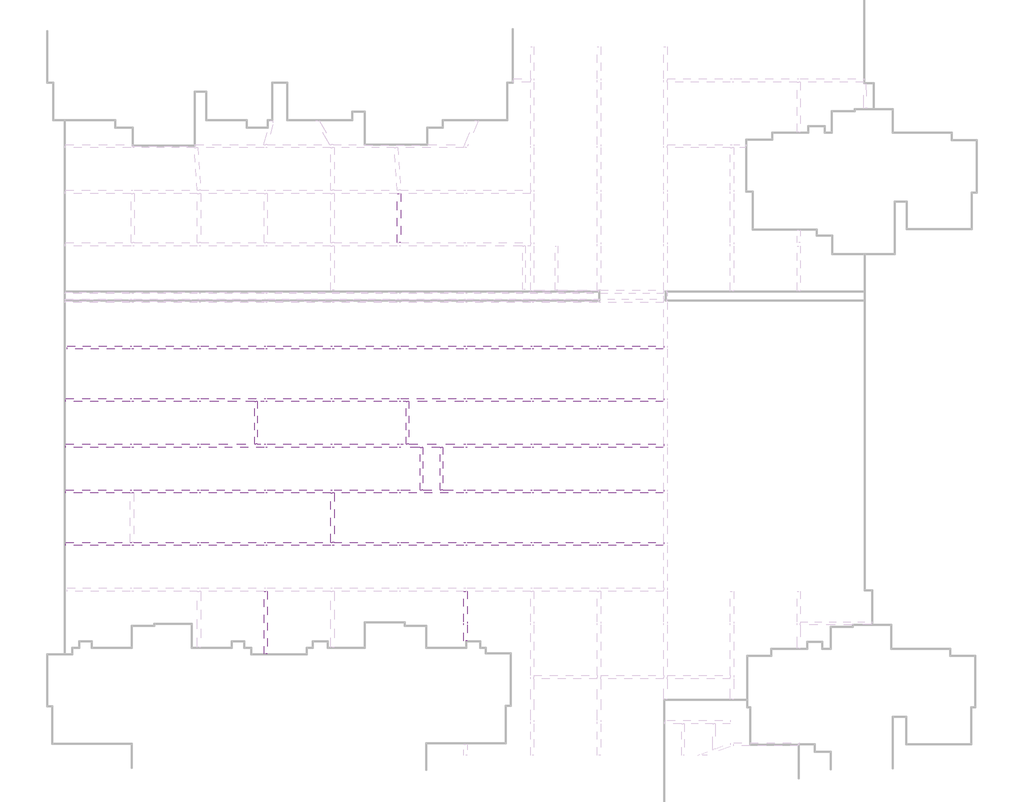
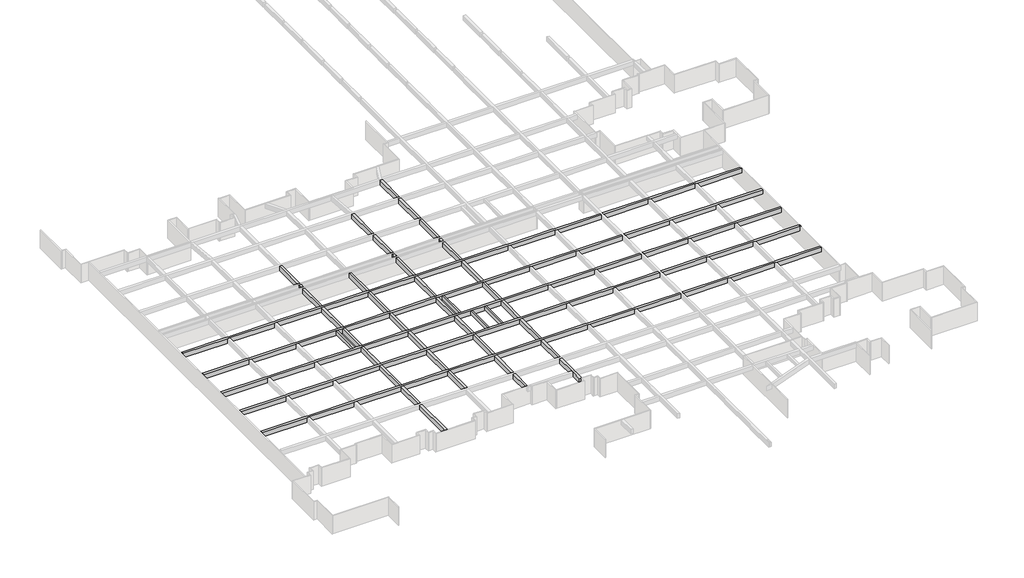
# One storey, part 9 of 14: 13 beams.
"""IFC4 building model written with IfcOpenShell, lengths in millimetres."""

from ifc_helpers import new_model, si_unit, frame, origin, place, context, project, spatial, polyline, outline, extrude, faceted_brep, element, save

model = new_model("IFC4")

# Units and contexts
model_context = context("Model", 3, world=origin())
ifc_project = project(units=[si_unit("LENGTHUNIT", "METRE", prefix="MILLI")], contexts=[model_context])

# Site, building, storey
site = spatial("IfcSite", under=ifc_project)
building = spatial("IfcBuilding", under=site)
storey = spatial("IfcBuildingStorey", under=building, Name="户型图", Elevation=0.0)

# Beams
placement = place(None, origin())
element("IfcBeam", 1, ObjectType="混凝土 - 矩形梁 : KL_beam", at=placement, inside=storey, context=model_context, shape_type="Brep", body=[
    faceted_brep([(-593917.6529954, -134659.4327531, 3300.0), (-593917.6529954, -134659.4327531, 2500.0), (-593917.6529954, -135059.4327531, 2500.0), (-593917.6529954, -135059.4327531, 3300.0), (-522267.6529954, -134659.4327531, 3300.0), (-522267.6529954, -135059.4327531, 3300.0), (-522267.6529954, -135059.4327531, 2500.0), (-522267.6529954, -134659.4327531, 2500.0), (-586331.2602569, -135059.4327531, 3300.0), (-585931.2602569, -135059.4327531, 3300.0), (-578267.6529954, -135059.4327531, 3300.0), (-577867.6529954, -135059.4327531, 3300.0), (-570267.6529954, -135059.4327531, 3300.0), (-569867.6529954, -135059.4327531, 3300.0), (-562267.6529954, -135059.4327531, 3300.0), (-561867.6529954, -135059.4327531, 3300.0), (-554267.6529954, -135059.4327531, 3300.0), (-553867.6529954, -135059.4327531, 3300.0), (-546267.6529954, -135059.4327531, 3300.0), (-545867.6529954, -135059.4327531, 3300.0), (-538267.6529954, -135059.4327531, 3300.0), (-537867.6529954, -135059.4327531, 3300.0), (-530267.6529954, -135059.4327531, 3300.0), (-529867.6529954, -135059.4327531, 3300.0), (-529867.6529954, -134659.4327531, 3300.0), (-530267.6529954, -134659.4327531, 3300.0), (-537867.6529954, -134659.4327531, 3300.0), (-538267.6529954, -134659.4327531, 3300.0), (-545867.6529954, -134659.4327531, 3300.0), (-546267.6529954, -134659.4327531, 3300.0), (-553867.6529954, -134659.4327531, 3300.0), (-554267.6529954, -134659.4327531, 3300.0), (-561867.6529954, -134659.4327531, 3300.0), (-562267.6529954, -134659.4327531, 3300.0), (-569867.6529954, -134659.4327531, 3300.0), (-570267.6529954, -134659.4327531, 3300.0), (-577867.6529954, -134659.4327531, 3300.0), (-578267.6529954, -134659.4327531, 3300.0), (-585931.2602569, -134659.4327531, 3300.0), (-586331.2602569, -134659.4327531, 3300.0), (-586331.2602569, -135059.4327531, 2500.0), (-585931.2602569, -135059.4327531, 2500.0), (-578267.6529954, -135059.4327531, 2500.0), (-577867.6529954, -135059.4327531, 2500.0), (-570267.6529954, -135059.4327531, 2500.0), (-569867.6529954, -135059.4327531, 2500.0), (-562267.6529954, -135059.4327531, 2500.0), (-561867.6529954, -135059.4327531, 2500.0), (-554267.6529954, -135059.4327531, 2500.0), (-553867.6529954, -135059.4327531, 2500.0), (-546267.6529954, -135059.4327531, 2500.0), (-545867.6529954, -135059.4327531, 2500.0), (-538267.6529954, -135059.4327531, 2500.0), (-537867.6529954, -135059.4327531, 2500.0), (-530267.6529954, -135059.4327531, 2500.0), (-529867.6529954, -135059.4327531, 2500.0), (-586331.2602569, -134659.4327531, 2500.0), (-585931.2602569, -134659.4327531, 2500.0), (-578267.6529954, -134659.4327531, 2500.0), (-577867.6529954, -134659.4327531, 2500.0), (-570267.6529954, -134659.4327531, 2500.0), (-569867.6529954, -134659.4327531, 2500.0), (-562267.6529954, -134659.4327531, 2500.0), (-561867.6529954, -134659.4327531, 2500.0), (-554267.6529954, -134659.4327531, 2500.0), (-553867.6529954, -134659.4327531, 2500.0), (-546267.6529954, -134659.4327531, 2500.0), (-545867.6529954, -134659.4327531, 2500.0), (-538267.6529954, -134659.4327531, 2500.0), (-537867.6529954, -134659.4327531, 2500.0), (-530267.6529954, -134659.4327531, 2500.0), (-529867.6529954, -134659.4327531, 2500.0)], [[[0, 1, 2, 3]], [[4, 5, 6, 7]], [[0, 3, 8, 9, 10, 11, 12, 13, 14, 15, 16, 17, 18, 19, 20, 21, 22, 23, 5, 4, 24, 25, 26, 27, 28, 29, 30, 31, 32, 33, 34, 35, 36, 37, 38, 39]], [[3, 2, 40, 41, 42, 43, 44, 45, 46, 47, 48, 49, 50, 51, 52, 53, 54, 55, 6, 5, 23, 22, 21, 20, 19, 18, 17, 16, 15, 14, 13, 12, 11, 10, 9, 8]], [[2, 1, 56, 57, 58, 59, 60, 61, 62, 63, 64, 65, 66, 67, 68, 69, 70, 71, 7, 6, 55, 54, 53, 52, 51, 50, 49, 48, 47, 46, 45, 44, 43, 42, 41, 40]], [[1, 0, 39, 38, 37, 36, 35, 34, 33, 32, 31, 30, 29, 28, 27, 26, 25, 24, 4, 7, 71, 70, 69, 68, 67, 66, 65, 64, 63, 62, 61, 60, 59, 58, 57, 56]]]),
    faceted_brep([(-498227.6529954, -135059.4327531, 3300.0), (-498227.6529954, -134659.4327531, 3300.0), (-505867.6529954, -134659.4327531, 3300.0), (-506267.6529954, -134659.4327531, 3300.0), (-513867.6529954, -134659.4327531, 3300.0), (-514267.6529954, -134659.4327531, 3300.0), (-521867.6529954, -134659.4327531, 3300.0), (-521867.6529954, -135059.4327531, 3300.0), (-514267.6529954, -135059.4327531, 3300.0), (-513867.6529954, -135059.4327531, 3300.0), (-506267.6529954, -135059.4327531, 3300.0), (-505867.6529954, -135059.4327531, 3300.0), (-498227.6529954, -135059.4327531, 2500.0), (-521867.6529954, -135059.4327531, 2500.0), (-514267.6529954, -135059.4327531, 2500.0), (-513867.6529954, -135059.4327531, 2500.0), (-506267.6529954, -135059.4327531, 2500.0), (-505867.6529954, -135059.4327531, 2500.0), (-498227.6529954, -134659.4327531, 2500.0), (-521867.6529954, -134659.4327531, 2500.0), (-514267.6529954, -134659.4327531, 2500.0), (-513867.6529954, -134659.4327531, 2500.0), (-506267.6529954, -134659.4327531, 2500.0), (-505867.6529954, -134659.4327531, 2500.0)], [[[0, 1, 2, 3, 4, 5, 6, 7, 8, 9, 10, 11]], [[12, 0, 11, 10, 9, 8, 7, 13, 14, 15, 16, 17]], [[18, 12, 17, 16, 15, 14, 13, 19, 20, 21, 22, 23]], [[1, 18, 23, 22, 21, 20, 19, 6, 5, 4, 3, 2]], [[1, 0, 12, 18]], [[7, 6, 19, 13]]]),
])
element("IfcBeam", 2, ObjectType="混凝土 - 矩形梁 : KL_beam", at=placement, inside=storey, context=model_context, shape_type="Brep", body=[
    faceted_brep([(-594067.6529954, -141359.4327531, 3300.0), (-594067.6529954, -140959.4327531, 3300.0), (-594067.6529954, -140959.4327531, 2500.0), (-594067.6529954, -141359.4327531, 2500.0), (-586331.2602569, -141359.4327531, 3300.0), (-585931.2602569, -141359.4327531, 3300.0), (-578267.6529954, -141359.4327531, 3300.0), (-577867.6529954, -141359.4327531, 3300.0), (-571417.6529954, -141359.4327531, 3300.0), (-571117.6529954, -141359.4327531, 3300.0), (-570267.6529954, -141359.4327531, 3300.0), (-569867.6529954, -141359.4327531, 3300.0), (-562267.6529954, -141359.4327531, 3300.0), (-561867.6529954, -141359.4327531, 3300.0), (-554267.6529954, -141359.4327531, 3300.0), (-553867.6529954, -141359.4327531, 3300.0), (-553217.6529954, -141359.4327531, 3300.0), (-552917.6529954, -141359.4327531, 3300.0), (-546267.6529954, -141359.4327531, 3300.0), (-545867.6529954, -141359.4327531, 3300.0), (-538267.6529954, -141359.4327531, 3300.0), (-537867.6529954, -141359.4327531, 3300.0), (-530267.6529954, -141359.4327531, 3300.0), (-529867.6529954, -141359.4327531, 3300.0), (-522267.6529954, -141359.4327531, 3300.0), (-522267.6529954, -140959.4327531, 3300.0), (-529867.6529954, -140959.4327531, 3300.0), (-530267.6529954, -140959.4327531, 3300.0), (-537867.6529954, -140959.4327531, 3300.0), (-538267.6529954, -140959.4327531, 3300.0), (-545867.6529954, -140959.4327531, 3300.0), (-546267.6529954, -140959.4327531, 3300.0), (-553867.6529954, -140959.4327531, 3300.0), (-554267.6529954, -140959.4327531, 3300.0), (-561867.6529954, -140959.4327531, 3300.0), (-562267.6529954, -140959.4327531, 3300.0), (-569867.6529954, -140959.4327531, 3300.0), (-570267.6529954, -140959.4327531, 3300.0), (-577867.6529954, -140959.4327531, 3300.0), (-578267.6529954, -140959.4327531, 3300.0), (-585931.2602569, -140959.4327531, 3300.0), (-586331.2602569, -140959.4327531, 3300.0), (-522267.6529954, -140959.4327531, 2500.0), (-529867.6529954, -140959.4327531, 2500.0), (-530267.6529954, -140959.4327531, 2500.0), (-537867.6529954, -140959.4327531, 2500.0), (-538267.6529954, -140959.4327531, 2500.0), (-545867.6529954, -140959.4327531, 2500.0), (-546267.6529954, -140959.4327531, 2500.0), (-553867.6529954, -140959.4327531, 2500.0), (-554267.6529954, -140959.4327531, 2500.0), (-561867.6529954, -140959.4327531, 2500.0), (-562267.6529954, -140959.4327531, 2500.0), (-569867.6529954, -140959.4327531, 2500.0), (-570267.6529954, -140959.4327531, 2500.0), (-577867.6529954, -140959.4327531, 2500.0), (-578267.6529954, -140959.4327531, 2500.0), (-585931.2602569, -140959.4327531, 2500.0), (-586331.2602569, -140959.4327531, 2500.0), (-522267.6529954, -141359.4327531, 2500.0), (-529867.6529954, -141359.4327531, 2500.0), (-530267.6529954, -141359.4327531, 2500.0), (-537867.6529954, -141359.4327531, 2500.0), (-538267.6529954, -141359.4327531, 2500.0), (-545867.6529954, -141359.4327531, 2500.0), (-546267.6529954, -141359.4327531, 2500.0), (-553867.6529954, -141359.4327531, 2500.0), (-554267.6529954, -141359.4327531, 2500.0), (-561867.6529954, -141359.4327531, 2500.0), (-562267.6529954, -141359.4327531, 2500.0), (-569867.6529954, -141359.4327531, 2500.0), (-570267.6529954, -141359.4327531, 2500.0), (-577867.6529954, -141359.4327531, 2500.0), (-578267.6529954, -141359.4327531, 2500.0), (-585931.2602569, -141359.4327531, 2500.0), (-586331.2602569, -141359.4327531, 2500.0)], [[[0, 1, 2, 3]], [[1, 0, 4, 5, 6, 7, 8, 9, 10, 11, 12, 13, 14, 15, 16, 17, 18, 19, 20, 21, 22, 23, 24, 25, 26, 27, 28, 29, 30, 31, 32, 33, 34, 35, 36, 37, 38, 39, 40, 41]], [[2, 1, 41, 40, 39, 38, 37, 36, 35, 34, 33, 32, 31, 30, 29, 28, 27, 26, 25, 42, 43, 44, 45, 46, 47, 48, 49, 50, 51, 52, 53, 54, 55, 56, 57, 58]], [[3, 2, 58, 57, 56, 55, 54, 53, 52, 51, 50, 49, 48, 47, 46, 45, 44, 43, 42, 59, 60, 61, 62, 63, 64, 65, 66, 67, 68, 69, 70, 71, 72, 73, 74, 75]], [[0, 3, 75, 74, 73, 72, 71, 70, 69, 68, 67, 66, 65, 64, 63, 62, 61, 60, 59, 24, 23, 22, 21, 20, 19, 18, 17, 16, 15, 14, 13, 12, 11, 10, 9, 8, 7, 6, 5, 4]], [[25, 24, 59, 42]]]),
    faceted_brep([(-498227.6529954, -140959.4327531, 3300.0), (-498227.6529954, -141359.4327531, 3300.0), (-498227.6529954, -141359.4327531, 2500.0), (-498227.6529954, -140959.4327531, 2500.0), (-521867.6529954, -141359.4327531, 3300.0), (-521867.6529954, -140959.4327531, 3300.0), (-521867.6529954, -140959.4327531, 2500.0), (-521867.6529954, -141359.4327531, 2500.0), (-505867.6529954, -140959.4327531, 3300.0), (-506267.6529954, -140959.4327531, 3300.0), (-513867.6529954, -140959.4327531, 3300.0), (-514267.6529954, -140959.4327531, 3300.0), (-514267.6529954, -141359.4327531, 3300.0), (-513867.6529954, -141359.4327531, 3300.0), (-506267.6529954, -141359.4327531, 3300.0), (-505867.6529954, -141359.4327531, 3300.0), (-505867.6529954, -140959.4327531, 2500.0), (-506267.6529954, -140959.4327531, 2500.0), (-513867.6529954, -140959.4327531, 2500.0), (-514267.6529954, -140959.4327531, 2500.0), (-505867.6529954, -141359.4327531, 2500.0), (-506267.6529954, -141359.4327531, 2500.0), (-513867.6529954, -141359.4327531, 2500.0), (-514267.6529954, -141359.4327531, 2500.0)], [[[0, 1, 2, 3]], [[4, 5, 6, 7]], [[1, 0, 8, 9, 10, 11, 5, 4, 12, 13, 14, 15]], [[0, 3, 16, 17, 18, 19, 6, 5, 11, 10, 9, 8]], [[3, 2, 20, 21, 22, 23, 7, 6, 19, 18, 17, 16]], [[2, 1, 15, 14, 13, 12, 4, 7, 23, 22, 21, 20]]]),
])
element("IfcBeam", 3, ObjectType="混凝土 - 矩形梁 : KL_beam", at=placement, inside=storey, context=model_context, shape_type="Brep", body=[
    faceted_brep([(-594067.6529954, -146459.4327531, 3300.0), (-594067.6529954, -146459.4327531, 2500.0), (-594067.6529954, -146859.4327531, 2500.0), (-594067.6529954, -146859.4327531, 3300.0), (-522267.6529954, -146459.4327531, 3300.0), (-522267.6529954, -146859.4327531, 3300.0), (-522267.6529954, -146859.4327531, 2500.0), (-522267.6529954, -146459.4327531, 2500.0), (-586331.2602569, -146859.4327531, 3300.0), (-585931.2602569, -146859.4327531, 3300.0), (-578267.6529954, -146859.4327531, 3300.0), (-577867.6529954, -146859.4327531, 3300.0), (-570267.6529954, -146859.4327531, 3300.0), (-569867.6529954, -146859.4327531, 3300.0), (-562267.6529954, -146859.4327531, 3300.0), (-561867.6529954, -146859.4327531, 3300.0), (-554267.6529954, -146859.4327531, 3300.0), (-553867.6529954, -146859.4327531, 3300.0), (-551517.6529954, -146859.4327531, 3300.0), (-551217.6529954, -146859.4327531, 3300.0), (-549117.6529954, -146859.4327531, 3300.0), (-548817.6529954, -146859.4327531, 3300.0), (-546267.6529954, -146859.4327531, 3300.0), (-545867.6529954, -146859.4327531, 3300.0), (-538267.6529954, -146859.4327531, 3300.0), (-537867.6529954, -146859.4327531, 3300.0), (-530267.6529954, -146859.4327531, 3300.0), (-529867.6529954, -146859.4327531, 3300.0), (-529867.6529954, -146459.4327531, 3300.0), (-530267.6529954, -146459.4327531, 3300.0), (-537867.6529954, -146459.4327531, 3300.0), (-538267.6529954, -146459.4327531, 3300.0), (-545867.6529954, -146459.4327531, 3300.0), (-546267.6529954, -146459.4327531, 3300.0), (-552917.6529954, -146459.4327531, 3300.0), (-553217.6529954, -146459.4327531, 3300.0), (-553867.6529954, -146459.4327531, 3300.0), (-554267.6529954, -146459.4327531, 3300.0), (-561867.6529954, -146459.4327531, 3300.0), (-562267.6529954, -146459.4327531, 3300.0), (-569867.6529954, -146459.4327531, 3300.0), (-570267.6529954, -146459.4327531, 3300.0), (-571117.6529954, -146459.4327531, 3300.0), (-571417.6529954, -146459.4327531, 3300.0), (-577867.6529954, -146459.4327531, 3300.0), (-578267.6529954, -146459.4327531, 3300.0), (-585931.2602569, -146459.4327531, 3300.0), (-586331.2602569, -146459.4327531, 3300.0), (-586331.2602569, -146859.4327531, 2500.0), (-585931.2602569, -146859.4327531, 2500.0), (-578267.6529954, -146859.4327531, 2500.0), (-577867.6529954, -146859.4327531, 2500.0), (-570267.6529954, -146859.4327531, 2500.0), (-569867.6529954, -146859.4327531, 2500.0), (-562267.6529954, -146859.4327531, 2500.0), (-561867.6529954, -146859.4327531, 2500.0), (-554267.6529954, -146859.4327531, 2500.0), (-553867.6529954, -146859.4327531, 2500.0), (-546267.6529954, -146859.4327531, 2500.0), (-545867.6529954, -146859.4327531, 2500.0), (-538267.6529954, -146859.4327531, 2500.0), (-537867.6529954, -146859.4327531, 2500.0), (-530267.6529954, -146859.4327531, 2500.0), (-529867.6529954, -146859.4327531, 2500.0), (-586331.2602569, -146459.4327531, 2500.0), (-585931.2602569, -146459.4327531, 2500.0), (-578267.6529954, -146459.4327531, 2500.0), (-577867.6529954, -146459.4327531, 2500.0), (-570267.6529954, -146459.4327531, 2500.0), (-569867.6529954, -146459.4327531, 2500.0), (-562267.6529954, -146459.4327531, 2500.0), (-561867.6529954, -146459.4327531, 2500.0), (-554267.6529954, -146459.4327531, 2500.0), (-553867.6529954, -146459.4327531, 2500.0), (-546267.6529954, -146459.4327531, 2500.0), (-545867.6529954, -146459.4327531, 2500.0), (-538267.6529954, -146459.4327531, 2500.0), (-537867.6529954, -146459.4327531, 2500.0), (-530267.6529954, -146459.4327531, 2500.0), (-529867.6529954, -146459.4327531, 2500.0)], [[[0, 1, 2, 3]], [[4, 5, 6, 7]], [[0, 3, 8, 9, 10, 11, 12, 13, 14, 15, 16, 17, 18, 19, 20, 21, 22, 23, 24, 25, 26, 27, 5, 4, 28, 29, 30, 31, 32, 33, 34, 35, 36, 37, 38, 39, 40, 41, 42, 43, 44, 45, 46, 47]], [[3, 2, 48, 49, 50, 51, 52, 53, 54, 55, 56, 57, 58, 59, 60, 61, 62, 63, 6, 5, 27, 26, 25, 24, 23, 22, 21, 20, 19, 18, 17, 16, 15, 14, 13, 12, 11, 10, 9, 8]], [[2, 1, 64, 65, 66, 67, 68, 69, 70, 71, 72, 73, 74, 75, 76, 77, 78, 79, 7, 6, 63, 62, 61, 60, 59, 58, 57, 56, 55, 54, 53, 52, 51, 50, 49, 48]], [[1, 0, 47, 46, 45, 44, 43, 42, 41, 40, 39, 38, 37, 36, 35, 34, 33, 32, 31, 30, 29, 28, 4, 7, 79, 78, 77, 76, 75, 74, 73, 72, 71, 70, 69, 68, 67, 66, 65, 64]]]),
    faceted_brep([(-498227.6529954, -146859.4327531, 3300.0), (-498227.6529954, -146459.4327531, 3300.0), (-505867.6529954, -146459.4327531, 3300.0), (-506267.6529954, -146459.4327531, 3300.0), (-513867.6529954, -146459.4327531, 3300.0), (-514267.6529954, -146459.4327531, 3300.0), (-521867.6529954, -146459.4327531, 3300.0), (-521867.6529954, -146859.4327531, 3300.0), (-514267.6529954, -146859.4327531, 3300.0), (-513867.6529954, -146859.4327531, 3300.0), (-506267.6529954, -146859.4327531, 3300.0), (-505867.6529954, -146859.4327531, 3300.0), (-498227.6529954, -146859.4327531, 2500.0), (-521867.6529954, -146859.4327531, 2500.0), (-514267.6529954, -146859.4327531, 2500.0), (-513867.6529954, -146859.4327531, 2500.0), (-506267.6529954, -146859.4327531, 2500.0), (-505867.6529954, -146859.4327531, 2500.0), (-498227.6529954, -146459.4327531, 2500.0), (-521867.6529954, -146459.4327531, 2500.0), (-514267.6529954, -146459.4327531, 2500.0), (-513867.6529954, -146459.4327531, 2500.0), (-506267.6529954, -146459.4327531, 2500.0), (-505867.6529954, -146459.4327531, 2500.0)], [[[0, 1, 2, 3, 4, 5, 6, 7, 8, 9, 10, 11]], [[12, 0, 11, 10, 9, 8, 7, 13, 14, 15, 16, 17]], [[18, 12, 17, 16, 15, 14, 13, 19, 20, 21, 22, 23]], [[1, 18, 23, 22, 21, 20, 19, 6, 5, 4, 3, 2]], [[1, 0, 12, 18]], [[7, 6, 19, 13]]]),
])
element("IfcBeam", 4, ObjectType="混凝土 - 矩形梁 : KL_beam", at=placement, inside=storey, context=model_context, shape_type="Brep", body=[
    faceted_brep([(-498067.6529954, -151959.4327531, 3300.0), (-498067.6529954, -152359.4327531, 3300.0), (-498067.6529954, -152359.4327531, 2500.0), (-498067.6529954, -151959.4327531, 2500.0), (-498107.6529954, -151959.4327531, 3300.0), (-498107.6529954, -152359.4327531, 3300.0), (-498107.6529954, -152359.4327531, 2500.0), (-498107.6529954, -151959.4327531, 2500.0)], [[[0, 1, 2, 3]], [[1, 0, 4, 5]], [[2, 1, 5, 6]], [[3, 2, 6, 7]], [[0, 3, 7, 4]], [[5, 4, 7, 6]]]),
    faceted_brep([(-594067.6529954, -151959.4327531, 3300.0), (-594067.6529954, -151959.4327531, 2500.0), (-594067.6529954, -152359.4327531, 2500.0), (-594067.6529954, -152359.4327531, 3300.0), (-522267.6529954, -151959.4327531, 3300.0), (-522267.6529954, -152359.4327531, 3300.0), (-522267.6529954, -152359.4327531, 2500.0), (-522267.6529954, -151959.4327531, 2500.0), (-586331.2602569, -152359.4327531, 3300.0), (-585931.2602569, -152359.4327531, 3300.0), (-578267.6529954, -152359.4327531, 3300.0), (-577867.6529954, -152359.4327531, 3300.0), (-570267.6529954, -152359.4327531, 3300.0), (-569867.6529954, -152359.4327531, 3300.0), (-562267.6529954, -152359.4327531, 3300.0), (-561867.6529954, -152359.4327531, 3300.0), (-554267.6529954, -152359.4327531, 3300.0), (-553867.6529954, -152359.4327531, 3300.0), (-546267.6529954, -152359.4327531, 3300.0), (-545867.6529954, -152359.4327531, 3300.0), (-538267.6529954, -152359.4327531, 3300.0), (-537867.6529954, -152359.4327531, 3300.0), (-530267.6529954, -152359.4327531, 3300.0), (-529867.6529954, -152359.4327531, 3300.0), (-529867.6529954, -151959.4327531, 3300.0), (-530267.6529954, -151959.4327531, 3300.0), (-537867.6529954, -151959.4327531, 3300.0), (-538267.6529954, -151959.4327531, 3300.0), (-545867.6529954, -151959.4327531, 3300.0), (-546267.6529954, -151959.4327531, 3300.0), (-548817.6529954, -151959.4327531, 3300.0), (-549117.6529954, -151959.4327531, 3300.0), (-551217.6529954, -151959.4327531, 3300.0), (-551517.6529954, -151959.4327531, 3300.0), (-553867.6529954, -151959.4327531, 3300.0), (-554267.6529954, -151959.4327531, 3300.0), (-561867.6529954, -151959.4327531, 3300.0), (-562267.6529954, -151959.4327531, 3300.0), (-569867.6529954, -151959.4327531, 3300.0), (-570267.6529954, -151959.4327531, 3300.0), (-577867.6529954, -151959.4327531, 3300.0), (-578267.6529954, -151959.4327531, 3300.0), (-585931.2602569, -151959.4327531, 3300.0), (-586331.2602569, -151959.4327531, 3300.0), (-586331.2602569, -152359.4327531, 2500.0), (-585931.2602569, -152359.4327531, 2500.0), (-578267.6529954, -152359.4327531, 2500.0), (-577867.6529954, -152359.4327531, 2500.0), (-570267.6529954, -152359.4327531, 2500.0), (-569867.6529954, -152359.4327531, 2500.0), (-562267.6529954, -152359.4327531, 2500.0), (-561867.6529954, -152359.4327531, 2500.0), (-554267.6529954, -152359.4327531, 2500.0), (-553867.6529954, -152359.4327531, 2500.0), (-546267.6529954, -152359.4327531, 2500.0), (-545867.6529954, -152359.4327531, 2500.0), (-538267.6529954, -152359.4327531, 2500.0), (-537867.6529954, -152359.4327531, 2500.0), (-530267.6529954, -152359.4327531, 2500.0), (-529867.6529954, -152359.4327531, 2500.0), (-586331.2602569, -151959.4327531, 2500.0), (-585931.2602569, -151959.4327531, 2500.0), (-578267.6529954, -151959.4327531, 2500.0), (-577867.6529954, -151959.4327531, 2500.0), (-570267.6529954, -151959.4327531, 2500.0), (-569867.6529954, -151959.4327531, 2500.0), (-562267.6529954, -151959.4327531, 2500.0), (-561867.6529954, -151959.4327531, 2500.0), (-554267.6529954, -151959.4327531, 2500.0), (-553867.6529954, -151959.4327531, 2500.0), (-546267.6529954, -151959.4327531, 2500.0), (-545867.6529954, -151959.4327531, 2500.0), (-538267.6529954, -151959.4327531, 2500.0), (-537867.6529954, -151959.4327531, 2500.0), (-530267.6529954, -151959.4327531, 2500.0), (-529867.6529954, -151959.4327531, 2500.0)], [[[0, 1, 2, 3]], [[4, 5, 6, 7]], [[0, 3, 8, 9, 10, 11, 12, 13, 14, 15, 16, 17, 18, 19, 20, 21, 22, 23, 5, 4, 24, 25, 26, 27, 28, 29, 30, 31, 32, 33, 34, 35, 36, 37, 38, 39, 40, 41, 42, 43]], [[3, 2, 44, 45, 46, 47, 48, 49, 50, 51, 52, 53, 54, 55, 56, 57, 58, 59, 6, 5, 23, 22, 21, 20, 19, 18, 17, 16, 15, 14, 13, 12, 11, 10, 9, 8]], [[2, 1, 60, 61, 62, 63, 64, 65, 66, 67, 68, 69, 70, 71, 72, 73, 74, 75, 7, 6, 59, 58, 57, 56, 55, 54, 53, 52, 51, 50, 49, 48, 47, 46, 45, 44]], [[1, 0, 43, 42, 41, 40, 39, 38, 37, 36, 35, 34, 33, 32, 31, 30, 29, 28, 27, 26, 25, 24, 4, 7, 75, 74, 73, 72, 71, 70, 69, 68, 67, 66, 65, 64, 63, 62, 61, 60]]]),
    faceted_brep([(-521867.6529954, -152359.4327531, 3300.0), (-521867.6529954, -151959.4327531, 3300.0), (-521867.6529954, -151959.4327531, 2500.0), (-521867.6529954, -152359.4327531, 2500.0), (-498227.6529954, -151959.4327531, 3300.0), (-498227.6529954, -152359.4327531, 3300.0), (-498227.6529954, -152359.4327531, 2500.0), (-498227.6529954, -151959.4327531, 2500.0), (-514267.6529954, -152359.4327531, 3300.0), (-513867.6529954, -152359.4327531, 3300.0), (-506267.6529954, -152359.4327531, 3300.0), (-505867.6529954, -152359.4327531, 3300.0), (-505867.6529954, -151959.4327531, 3300.0), (-506267.6529954, -151959.4327531, 3300.0), (-513867.6529954, -151959.4327531, 3300.0), (-514267.6529954, -151959.4327531, 3300.0), (-514267.6529954, -152359.4327531, 2500.0), (-513867.6529954, -152359.4327531, 2500.0), (-506267.6529954, -152359.4327531, 2500.0), (-505867.6529954, -152359.4327531, 2500.0), (-514267.6529954, -151959.4327531, 2500.0), (-513867.6529954, -151959.4327531, 2500.0), (-506267.6529954, -151959.4327531, 2500.0), (-505867.6529954, -151959.4327531, 2500.0)], [[[0, 1, 2, 3]], [[4, 5, 6, 7]], [[1, 0, 8, 9, 10, 11, 5, 4, 12, 13, 14, 15]], [[0, 3, 16, 17, 18, 19, 6, 5, 11, 10, 9, 8]], [[3, 2, 20, 21, 22, 23, 7, 6, 19, 18, 17, 16]], [[2, 1, 15, 14, 13, 12, 4, 7, 23, 22, 21, 20]]]),
])
element("IfcBeam", 5, ObjectType="混凝土 - 矩形梁 : KL_beam", at=placement, inside=storey, context=model_context, shape_type="Brep", body=[
    faceted_brep([(-594067.6529954, -158659.4327531, 3300.0), (-594067.6529954, -158259.4327531, 3300.0), (-594067.6529954, -158259.4327531, 2500.0), (-594067.6529954, -158659.4327531, 2500.0), (-586331.2602569, -158659.4327531, 3300.0), (-585931.2602569, -158659.4327531, 3300.0), (-578267.6529954, -158659.4327531, 3300.0), (-577867.6529954, -158659.4327531, 3300.0), (-570267.6529954, -158659.4327531, 3300.0), (-569867.6529954, -158659.4327531, 3300.0), (-562267.6529954, -158659.4327531, 3300.0), (-561867.6529954, -158659.4327531, 3300.0), (-554267.6529954, -158659.4327531, 3300.0), (-553867.6529954, -158659.4327531, 3300.0), (-546267.6529954, -158659.4327531, 3300.0), (-545867.6529954, -158659.4327531, 3300.0), (-538267.6529954, -158659.4327531, 3300.0), (-537867.6529954, -158659.4327531, 3300.0), (-530267.6529954, -158659.4327531, 3300.0), (-529867.6529954, -158659.4327531, 3300.0), (-522267.6529954, -158659.4327531, 3300.0), (-522267.6529954, -158259.4327531, 3300.0), (-529867.6529954, -158259.4327531, 3300.0), (-530267.6529954, -158259.4327531, 3300.0), (-537867.6529954, -158259.4327531, 3300.0), (-538267.6529954, -158259.4327531, 3300.0), (-545867.6529954, -158259.4327531, 3300.0), (-546267.6529954, -158259.4327531, 3300.0), (-553867.6529954, -158259.4327531, 3300.0), (-554267.6529954, -158259.4327531, 3300.0), (-561867.6529954, -158259.4327531, 3300.0), (-562267.6529954, -158259.4327531, 3300.0), (-569867.6529954, -158259.4327531, 3300.0), (-570267.6529954, -158259.4327531, 3300.0), (-577867.6529954, -158259.4327531, 3300.0), (-578267.6529954, -158259.4327531, 3300.0), (-585931.2602569, -158259.4327531, 3300.0), (-586331.2602569, -158259.4327531, 3300.0), (-522267.6529954, -158259.4327531, 2500.0), (-529867.6529954, -158259.4327531, 2500.0), (-530267.6529954, -158259.4327531, 2500.0), (-537867.6529954, -158259.4327531, 2500.0), (-538267.6529954, -158259.4327531, 2500.0), (-545867.6529954, -158259.4327531, 2500.0), (-546267.6529954, -158259.4327531, 2500.0), (-553867.6529954, -158259.4327531, 2500.0), (-554267.6529954, -158259.4327531, 2500.0), (-561867.6529954, -158259.4327531, 2500.0), (-562267.6529954, -158259.4327531, 2500.0), (-569867.6529954, -158259.4327531, 2500.0), (-570267.6529954, -158259.4327531, 2500.0), (-577867.6529954, -158259.4327531, 2500.0), (-578267.6529954, -158259.4327531, 2500.0), (-585931.2602569, -158259.4327531, 2500.0), (-586331.2602569, -158259.4327531, 2500.0), (-522267.6529954, -158659.4327531, 2500.0), (-529867.6529954, -158659.4327531, 2500.0), (-530267.6529954, -158659.4327531, 2500.0), (-537867.6529954, -158659.4327531, 2500.0), (-538267.6529954, -158659.4327531, 2500.0), (-545867.6529954, -158659.4327531, 2500.0), (-546267.6529954, -158659.4327531, 2500.0), (-553867.6529954, -158659.4327531, 2500.0), (-554267.6529954, -158659.4327531, 2500.0), (-561867.6529954, -158659.4327531, 2500.0), (-562267.6529954, -158659.4327531, 2500.0), (-569867.6529954, -158659.4327531, 2500.0), (-570267.6529954, -158659.4327531, 2500.0), (-577867.6529954, -158659.4327531, 2500.0), (-578267.6529954, -158659.4327531, 2500.0), (-585931.2602569, -158659.4327531, 2500.0), (-586331.2602569, -158659.4327531, 2500.0)], [[[0, 1, 2, 3]], [[1, 0, 4, 5, 6, 7, 8, 9, 10, 11, 12, 13, 14, 15, 16, 17, 18, 19, 20, 21, 22, 23, 24, 25, 26, 27, 28, 29, 30, 31, 32, 33, 34, 35, 36, 37]], [[2, 1, 37, 36, 35, 34, 33, 32, 31, 30, 29, 28, 27, 26, 25, 24, 23, 22, 21, 38, 39, 40, 41, 42, 43, 44, 45, 46, 47, 48, 49, 50, 51, 52, 53, 54]], [[3, 2, 54, 53, 52, 51, 50, 49, 48, 47, 46, 45, 44, 43, 42, 41, 40, 39, 38, 55, 56, 57, 58, 59, 60, 61, 62, 63, 64, 65, 66, 67, 68, 69, 70, 71]], [[0, 3, 71, 70, 69, 68, 67, 66, 65, 64, 63, 62, 61, 60, 59, 58, 57, 56, 55, 20, 19, 18, 17, 16, 15, 14, 13, 12, 11, 10, 9, 8, 7, 6, 5, 4]], [[21, 20, 55, 38]]]),
    faceted_brep([(-498227.6529954, -158259.4327531, 3300.0), (-498227.6529954, -158659.4327531, 3300.0), (-498227.6529954, -158659.4327531, 2500.0), (-498227.6529954, -158259.4327531, 2500.0), (-521867.6529954, -158659.4327531, 3300.0), (-521867.6529954, -158259.4327531, 3300.0), (-521867.6529954, -158259.4327531, 2500.0), (-521867.6529954, -158659.4327531, 2500.0), (-505867.6529954, -158259.4327531, 3300.0), (-506267.6529954, -158259.4327531, 3300.0), (-513867.6529954, -158259.4327531, 3300.0), (-514267.6529954, -158259.4327531, 3300.0), (-514267.6529954, -158659.4327531, 3300.0), (-513867.6529954, -158659.4327531, 3300.0), (-506267.6529954, -158659.4327531, 3300.0), (-505867.6529954, -158659.4327531, 3300.0), (-505867.6529954, -158259.4327531, 2500.0), (-506267.6529954, -158259.4327531, 2500.0), (-513867.6529954, -158259.4327531, 2500.0), (-514267.6529954, -158259.4327531, 2500.0), (-505867.6529954, -158659.4327531, 2500.0), (-506267.6529954, -158659.4327531, 2500.0), (-513867.6529954, -158659.4327531, 2500.0), (-514267.6529954, -158659.4327531, 2500.0)], [[[0, 1, 2, 3]], [[4, 5, 6, 7]], [[1, 0, 8, 9, 10, 11, 5, 4, 12, 13, 14, 15]], [[0, 3, 16, 17, 18, 19, 6, 5, 11, 10, 9, 8]], [[3, 2, 20, 21, 22, 23, 7, 6, 19, 18, 17, 16]], [[2, 1, 15, 14, 13, 12, 4, 7, 23, 22, 21, 20]]]),
])
element("IfcBeam", 6, ObjectType="混凝土 - 矩形梁 : KL_beam", at=placement, inside=storey, context=model_context, shape_type="SweptSolid", body=[
    extrude(outline(polyline([(-569867.6529954, -171682.856538), (-570267.6529954, -171682.856538), (-570267.6529954, -164159.4327531), (-569867.6529954, -164159.4327531), (-569867.6529954, -171682.856538)])), frame((0.0, 0.0, 2500.0), z_axis=(0.0, 0.0, 1.0), x_axis=(1.0, 0.0, 0.0)), (0.0, 0.0, 1.0), 800.0),
    extrude(outline(polyline([(-570267.6529954, -122659.4327531), (-569867.6529954, -122659.4327531), (-569867.6529954, -127959.4327532), (-570267.6529954, -127959.4327532), (-570267.6529954, -122659.4327531)])), frame((0.0, 0.0, 2500.0), z_axis=(0.0, 0.0, 1.0), x_axis=(1.0, 0.0, 0.0)), (0.0, 0.0, 1.0), 800.0),
    extrude(outline(polyline([(-570267.6529954, -128359.4327532), (-569867.6529954, -128359.4327532), (-569867.6529954, -129034.4327531), (-570267.6529954, -129034.4327531), (-570267.6529954, -128359.4327532)])), frame((0.0, 0.0, 2500.0), z_axis=(0.0, 0.0, 1.0), x_axis=(1.0, 0.0, 0.0)), (0.0, 0.0, 1.0), 800.0),
    extrude(outline(polyline([(-570267.6529954, -129434.4327531), (-569867.6529954, -129434.4327531), (-569867.6529954, -134659.4327531), (-570267.6529954, -134659.4327531), (-570267.6529954, -129434.4327531)])), frame((0.0, 0.0, 2500.0), z_axis=(0.0, 0.0, 1.0), x_axis=(1.0, 0.0, 0.0)), (0.0, 0.0, 1.0), 800.0),
    extrude(outline(polyline([(-570267.6529954, -135059.4327531), (-569867.6529954, -135059.4327531), (-569867.6529954, -140959.4327531), (-570267.6529954, -140959.4327531), (-570267.6529954, -135059.4327531)])), frame((0.0, 0.0, 2500.0), z_axis=(0.0, 0.0, 1.0), x_axis=(1.0, 0.0, 0.0)), (0.0, 0.0, 1.0), 800.0),
    extrude(outline(polyline([(-570267.6529954, -141359.4327531), (-569867.6529954, -141359.4327531), (-569867.6529954, -146459.4327531), (-570267.6529954, -146459.4327531), (-570267.6529954, -141359.4327531)])), frame((0.0, 0.0, 2500.0), z_axis=(0.0, 0.0, 1.0), x_axis=(1.0, 0.0, 0.0)), (0.0, 0.0, 1.0), 800.0),
    extrude(outline(polyline([(-570267.6529954, -146859.4327531), (-569867.6529954, -146859.4327531), (-569867.6529954, -151959.4327531), (-570267.6529954, -151959.4327531), (-570267.6529954, -146859.4327531)])), frame((0.0, 0.0, 2500.0), z_axis=(0.0, 0.0, 1.0), x_axis=(1.0, 0.0, 0.0)), (0.0, 0.0, 1.0), 800.0),
    extrude(outline(polyline([(-570267.6529954, -152359.4327531), (-569867.6529954, -152359.4327531), (-569867.6529954, -158259.4327531), (-570267.6529954, -158259.4327531), (-570267.6529954, -152359.4327531)])), frame((0.0, 0.0, 2500.0), z_axis=(0.0, 0.0, 1.0), x_axis=(1.0, 0.0, 0.0)), (0.0, 0.0, 1.0), 800.0),
    extrude(outline(polyline([(-570267.6529954, -158659.4327531), (-569867.6529954, -158659.4327531), (-569867.6529954, -163759.4327531), (-570267.6529954, -163759.4327531), (-570267.6529954, -158659.4327531)])), frame((0.0, 0.0, 2500.0), z_axis=(0.0, 0.0, 1.0), x_axis=(1.0, 0.0, 0.0)), (0.0, 0.0, 1.0), 800.0),
])
element("IfcBeam", 7, ObjectType="混凝土 - 矩形梁 : KL_beam", at=placement, inside=storey, context=model_context, shape_type="Brep", body=[
    faceted_brep([(-553867.6529954, -116357.5126628, 3300.0), (-554267.6529954, -116357.5126628, 3300.0), (-554267.6529954, -122259.4327531, 3300.0), (-553867.6529954, -122259.4327531, 3300.0), (-554267.6529954, -116357.5126628, 2500.0), (-554267.6529954, -122259.4327531, 2500.0), (-553867.6529954, -116357.5126628, 2500.0), (-553867.6529954, -122259.4327531, 2500.0)], [[[0, 1, 2, 3]], [[1, 4, 5, 2]], [[4, 6, 7, 5]], [[6, 0, 3, 7]], [[1, 0, 6, 4]], [[3, 2, 5, 7]]]),
    faceted_brep([(-553867.6529954, -167832.8565288, 3300.0), (-554267.6529954, -167832.8565288, 3300.0), (-554267.6529954, -167832.8565288, 2500.0), (-553867.6529954, -167832.8565288, 2500.0), (-554267.6529954, -164159.4327531, 3300.0), (-553867.6529954, -164159.4327531, 3300.0), (-553867.6529954, -164159.4327531, 2500.0), (-554267.6529954, -164159.4327531, 2500.0), (-553867.6529954, -167800.507479, 3300.0), (-553867.6529954, -167800.507479, 2500.0)], [[[0, 1, 2, 3]], [[4, 5, 6, 7]], [[1, 0, 8, 5, 4]], [[2, 1, 4, 7]], [[3, 2, 7, 6, 9]], [[0, 3, 9, 6, 5, 8]]]),
    faceted_brep([(-554267.6529954, -122659.4327531, 3300.0), (-553867.6529954, -122659.4327531, 3300.0), (-553867.6529954, -122659.4327531, 2500.0), (-554267.6529954, -122659.4327531, 2500.0), (-553867.6529954, -127959.4327532, 3300.0), (-554267.6529954, -127959.4327532, 3300.0), (-554267.6529954, -127959.4327532, 2500.0), (-553867.6529954, -127959.4327532, 2500.0)], [[[0, 1, 2, 3]], [[4, 5, 6, 7]], [[1, 0, 5, 4]], [[0, 3, 6, 5]], [[3, 2, 7, 6]], [[2, 1, 4, 7]]]),
    faceted_brep([(-553867.6529954, -128359.4327532, 3300.0), (-554267.6529954, -128359.4327532, 3300.0), (-554267.6529954, -129034.4327531, 3300.0), (-553867.6529954, -129034.4327531, 3300.0), (-554267.6529954, -128359.4327532, 2500.0), (-554267.6529954, -129034.4327531, 2500.0), (-553867.6529954, -128359.4327532, 2500.0), (-553867.6529954, -129034.4327531, 2500.0)], [[[0, 1, 2, 3]], [[1, 4, 5, 2]], [[4, 6, 7, 5]], [[6, 0, 3, 7]], [[1, 0, 6, 4]], [[3, 2, 5, 7]]]),
    faceted_brep([(-554267.6529954, -129434.4327531, 3300.0), (-553867.6529954, -129434.4327531, 3300.0), (-553867.6529954, -129434.4327531, 2500.0), (-554267.6529954, -129434.4327531, 2500.0), (-553867.6529954, -134659.4327531, 3300.0), (-554267.6529954, -134659.4327531, 3300.0), (-554267.6529954, -134659.4327531, 2500.0), (-553867.6529954, -134659.4327531, 2500.0)], [[[0, 1, 2, 3]], [[4, 5, 6, 7]], [[1, 0, 5, 4]], [[0, 3, 6, 5]], [[3, 2, 7, 6]], [[2, 1, 4, 7]]]),
    faceted_brep([(-553867.6529954, -135059.4327531, 3300.0), (-554267.6529954, -135059.4327531, 3300.0), (-554267.6529954, -140959.4327531, 3300.0), (-553867.6529954, -140959.4327531, 3300.0), (-554267.6529954, -135059.4327531, 2500.0), (-554267.6529954, -140959.4327531, 2500.0), (-553867.6529954, -135059.4327531, 2500.0), (-553867.6529954, -140959.4327531, 2500.0)], [[[0, 1, 2, 3]], [[1, 4, 5, 2]], [[4, 6, 7, 5]], [[6, 0, 3, 7]], [[1, 0, 6, 4]], [[3, 2, 5, 7]]]),
    faceted_brep([(-554267.6529954, -141359.4327531, 3300.0), (-553867.6529954, -141359.4327531, 3300.0), (-553867.6529954, -141359.4327531, 2500.0), (-554267.6529954, -141359.4327531, 2500.0), (-553867.6529954, -146459.4327531, 3300.0), (-554267.6529954, -146459.4327531, 3300.0), (-554267.6529954, -146459.4327531, 2500.0), (-553867.6529954, -146459.4327531, 2500.0)], [[[0, 1, 2, 3]], [[4, 5, 6, 7]], [[1, 0, 5, 4]], [[0, 3, 6, 5]], [[3, 2, 7, 6]], [[2, 1, 4, 7]]]),
    faceted_brep([(-553867.6529954, -146859.4327531, 3300.0), (-554267.6529954, -146859.4327531, 3300.0), (-554267.6529954, -151959.4327531, 3300.0), (-553867.6529954, -151959.4327531, 3300.0), (-554267.6529954, -146859.4327531, 2500.0), (-554267.6529954, -151959.4327531, 2500.0), (-553867.6529954, -146859.4327531, 2500.0), (-553867.6529954, -151959.4327531, 2500.0)], [[[0, 1, 2, 3]], [[1, 4, 5, 2]], [[4, 6, 7, 5]], [[6, 0, 3, 7]], [[1, 0, 6, 4]], [[3, 2, 5, 7]]]),
    faceted_brep([(-554267.6529954, -152359.4327531, 3300.0), (-553867.6529954, -152359.4327531, 3300.0), (-553867.6529954, -152359.4327531, 2500.0), (-554267.6529954, -152359.4327531, 2500.0), (-553867.6529954, -158259.4327531, 3300.0), (-554267.6529954, -158259.4327531, 3300.0), (-554267.6529954, -158259.4327531, 2500.0), (-553867.6529954, -158259.4327531, 2500.0)], [[[0, 1, 2, 3]], [[4, 5, 6, 7]], [[1, 0, 5, 4]], [[0, 3, 6, 5]], [[3, 2, 7, 6]], [[2, 1, 4, 7]]]),
    faceted_brep([(-553867.6529954, -158659.4327531, 3300.0), (-554267.6529954, -158659.4327531, 3300.0), (-554267.6529954, -163759.4327531, 3300.0), (-553867.6529954, -163759.4327531, 3300.0), (-554267.6529954, -158659.4327531, 2500.0), (-554267.6529954, -163759.4327531, 2500.0), (-553867.6529954, -158659.4327531, 2500.0), (-553867.6529954, -163759.4327531, 2500.0)], [[[0, 1, 2, 3]], [[1, 4, 5, 2]], [[4, 6, 7, 5]], [[6, 0, 3, 7]], [[1, 0, 6, 4]], [[3, 2, 5, 7]]]),
])
element("IfcBeam", 8, ObjectType="混凝土 - 矩形梁 : KL_beam", at=placement, inside=storey, context=model_context, shape_type="Brep", body=[
    faceted_brep([(-546267.6529954, -170082.6446455, 3300.0), (-546267.6529954, -170082.6446455, 2500.0), (-545867.6529954, -170082.6446455, 2500.0), (-545867.6529954, -170082.6446455, 3300.0), (-545867.6529954, -164159.4327531, 3300.0), (-545867.6529954, -164159.4327531, 2500.0), (-546267.6529954, -164159.4327531, 2500.0), (-546267.6529954, -164159.4327531, 3300.0), (-545867.6529954, -168200.507479, 2500.0), (-545867.6529954, -167800.507479, 2500.0), (-545867.6529954, -167800.507479, 3300.0), (-545867.6529954, -168200.507479, 3300.0), (-546267.6529954, -167800.507479, 3300.0), (-546267.6529954, -168200.507479, 3300.0), (-546267.6529954, -168200.507479, 2500.0), (-546267.6529954, -167800.507479, 2500.0)], [[[0, 1, 2, 3]], [[4, 5, 6, 7]], [[3, 2, 8, 9, 5, 4, 10, 11]], [[0, 3, 11, 10, 4, 7, 12, 13]], [[2, 1, 14, 15, 6, 5, 9, 8]], [[1, 0, 13, 12, 7, 6, 15, 14]]]),
    faceted_brep([(-545867.6529954, -110859.4327531, 2500.0), (-545867.6529954, -110859.4327531, 3300.0), (-545867.6529954, -115957.5126628, 3300.0), (-545867.6529954, -115957.5126628, 2500.0), (-545935.2758832, -110859.4327531, 3300.0), (-546267.6529954, -110859.4327531, 3300.0), (-546267.6529954, -115957.5126628, 3300.0), (-546267.6529954, -110859.4327531, 2500.0), (-545935.2758832, -110859.4327531, 2500.0), (-546267.6529954, -115957.5126628, 2500.0)], [[[0, 1, 2, 3]], [[1, 4, 5, 6, 2]], [[7, 8, 0, 3, 9]], [[5, 7, 9, 6]], [[1, 0, 8, 7, 5, 4]], [[3, 2, 6, 9]]]),
    faceted_brep([(-545867.6529954, -116357.5126628, 3300.0), (-545867.6529954, -116357.5126628, 2500.0), (-546267.6529954, -116357.5126628, 2500.0), (-546267.6529954, -116357.5126628, 3300.0), (-545867.6529954, -122259.4327531, 3300.0), (-545867.6529954, -122259.4327531, 2500.0), (-546267.6529954, -122259.4327531, 3300.0), (-546267.6529954, -122259.4327531, 2500.0)], [[[0, 1, 2, 3]], [[1, 0, 4, 5]], [[0, 3, 6, 4]], [[2, 1, 5, 7]], [[3, 2, 7, 6]], [[5, 4, 6, 7]]]),
    faceted_brep([(-545867.6529954, -122659.4327531, 3300.0), (-545867.6529954, -122659.4327531, 2500.0), (-546267.6529954, -122659.4327531, 2500.0), (-546267.6529954, -122659.4327531, 3300.0), (-545867.6529954, -127959.4327532, 3300.0), (-545867.6529954, -127959.4327532, 2500.0), (-546267.6529954, -127959.4327532, 3300.0), (-546267.6529954, -127959.4327532, 2500.0)], [[[0, 1, 2, 3]], [[1, 0, 4, 5]], [[0, 3, 6, 4]], [[2, 1, 5, 7]], [[3, 2, 7, 6]], [[5, 4, 6, 7]]]),
    faceted_brep([(-545867.6529954, -128359.4327532, 3300.0), (-545867.6529954, -128359.4327532, 2500.0), (-546267.6529954, -128359.4327532, 2500.0), (-546267.6529954, -128359.4327532, 3300.0), (-545867.6529954, -129034.4327531, 3300.0), (-545867.6529954, -129034.4327531, 2500.0), (-546267.6529954, -129034.4327531, 3300.0), (-546267.6529954, -129034.4327531, 2500.0)], [[[0, 1, 2, 3]], [[1, 0, 4, 5]], [[0, 3, 6, 4]], [[2, 1, 5, 7]], [[3, 2, 7, 6]], [[5, 4, 6, 7]]]),
    faceted_brep([(-545867.6529954, -129434.4327531, 3300.0), (-545867.6529954, -129434.4327531, 2500.0), (-546267.6529954, -129434.4327531, 2500.0), (-546267.6529954, -129434.4327531, 3300.0), (-545867.6529954, -134659.4327531, 3300.0), (-545867.6529954, -134659.4327531, 2500.0), (-546267.6529954, -134659.4327531, 3300.0), (-546267.6529954, -134659.4327531, 2500.0)], [[[0, 1, 2, 3]], [[1, 0, 4, 5]], [[0, 3, 6, 4]], [[2, 1, 5, 7]], [[3, 2, 7, 6]], [[5, 4, 6, 7]]]),
    faceted_brep([(-545867.6529954, -135059.4327531, 3300.0), (-545867.6529954, -135059.4327531, 2500.0), (-546267.6529954, -135059.4327531, 2500.0), (-546267.6529954, -135059.4327531, 3300.0), (-545867.6529954, -140959.4327531, 3300.0), (-545867.6529954, -140959.4327531, 2500.0), (-546267.6529954, -140959.4327531, 3300.0), (-546267.6529954, -140959.4327531, 2500.0)], [[[0, 1, 2, 3]], [[1, 0, 4, 5]], [[0, 3, 6, 4]], [[2, 1, 5, 7]], [[3, 2, 7, 6]], [[5, 4, 6, 7]]]),
    faceted_brep([(-545867.6529954, -141359.4327531, 3300.0), (-545867.6529954, -141359.4327531, 2500.0), (-546267.6529954, -141359.4327531, 2500.0), (-546267.6529954, -141359.4327531, 3300.0), (-545867.6529954, -146459.4327531, 3300.0), (-545867.6529954, -146459.4327531, 2500.0), (-546267.6529954, -146459.4327531, 3300.0), (-546267.6529954, -146459.4327531, 2500.0)], [[[0, 1, 2, 3]], [[1, 0, 4, 5]], [[0, 3, 6, 4]], [[2, 1, 5, 7]], [[3, 2, 7, 6]], [[5, 4, 6, 7]]]),
    faceted_brep([(-545867.6529954, -146859.4327531, 3300.0), (-545867.6529954, -146859.4327531, 2500.0), (-546267.6529954, -146859.4327531, 2500.0), (-546267.6529954, -146859.4327531, 3300.0), (-545867.6529954, -151959.4327531, 3300.0), (-545867.6529954, -151959.4327531, 2500.0), (-546267.6529954, -151959.4327531, 3300.0), (-546267.6529954, -151959.4327531, 2500.0)], [[[0, 1, 2, 3]], [[1, 0, 4, 5]], [[0, 3, 6, 4]], [[2, 1, 5, 7]], [[3, 2, 7, 6]], [[5, 4, 6, 7]]]),
    faceted_brep([(-545867.6529954, -152359.4327531, 3300.0), (-545867.6529954, -152359.4327531, 2500.0), (-546267.6529954, -152359.4327531, 2500.0), (-546267.6529954, -152359.4327531, 3300.0), (-545867.6529954, -158259.4327531, 3300.0), (-545867.6529954, -158259.4327531, 2500.0), (-546267.6529954, -158259.4327531, 3300.0), (-546267.6529954, -158259.4327531, 2500.0)], [[[0, 1, 2, 3]], [[1, 0, 4, 5]], [[0, 3, 6, 4]], [[2, 1, 5, 7]], [[3, 2, 7, 6]], [[5, 4, 6, 7]]]),
    faceted_brep([(-545867.6529954, -158659.4327531, 3300.0), (-545867.6529954, -158659.4327531, 2500.0), (-546267.6529954, -158659.4327531, 2500.0), (-546267.6529954, -158659.4327531, 3300.0), (-545867.6529954, -163759.4327531, 3300.0), (-545867.6529954, -163759.4327531, 2500.0), (-546267.6529954, -163759.4327531, 3300.0), (-546267.6529954, -163759.4327531, 2500.0)], [[[0, 1, 2, 3]], [[1, 0, 4, 5]], [[0, 3, 6, 4]], [[2, 1, 5, 7]], [[3, 2, 7, 6]], [[5, 4, 6, 7]]]),
])
element("IfcBeam", 9, ObjectType="混凝土 - 矩形梁 : KL_beam", at=placement, inside=storey, context=model_context, shape_type="SweptSolid", body=[
    extrude(outline(polyline([(-562267.6529954, -129434.4327531), (-561867.6529954, -129434.4327531), (-561867.6529954, -134659.4327531), (-562267.6529954, -134659.4327531), (-562267.6529954, -129434.4327531)])), frame((0.0, 0.0, 2500.0), z_axis=(0.0, 0.0, 1.0), x_axis=(1.0, 0.0, 0.0)), (0.0, 0.0, 1.0), 800.0),
    extrude(outline(polyline([(-561867.6529954, -163759.4327531), (-562267.6529954, -163759.4327531), (-562267.6529954, -158659.4327531), (-561867.6529954, -158659.4327531), (-561867.6529954, -163759.4327531)])), frame((0.0, 0.0, 2500.0), z_axis=(0.0, 0.0, 1.0), x_axis=(1.0, 0.0, 0.0)), (0.0, 0.0, 1.0), 800.0),
    extrude(outline(polyline([(-562267.6529954, -135059.4327531), (-561867.6529954, -135059.4327531), (-561867.6529954, -140959.4327531), (-562267.6529954, -140959.4327531), (-562267.6529954, -135059.4327531)])), frame((0.0, 0.0, 2500.0), z_axis=(0.0, 0.0, 1.0), x_axis=(1.0, 0.0, 0.0)), (0.0, 0.0, 1.0), 800.0),
    extrude(outline(polyline([(-562267.6529954, -141359.4327531), (-561867.6529954, -141359.4327531), (-561867.6529954, -146459.4327531), (-562267.6529954, -146459.4327531), (-562267.6529954, -141359.4327531)])), frame((0.0, 0.0, 2500.0), z_axis=(0.0, 0.0, 1.0), x_axis=(1.0, 0.0, 0.0)), (0.0, 0.0, 1.0), 800.0),
    extrude(outline(polyline([(-562267.6529954, -146859.4327531), (-561867.6529954, -146859.4327531), (-561867.6529954, -151959.4327531), (-562267.6529954, -151959.4327531), (-562267.6529954, -146859.4327531)])), frame((0.0, 0.0, 2500.0), z_axis=(0.0, 0.0, 1.0), x_axis=(1.0, 0.0, 0.0)), (0.0, 0.0, 1.0), 800.0),
    extrude(outline(polyline([(-562267.6529954, -152359.4327531), (-561867.6529954, -152359.4327531), (-561867.6529954, -158259.4327531), (-562267.6529954, -158259.4327531), (-562267.6529954, -152359.4327531)])), frame((0.0, 0.0, 2500.0), z_axis=(0.0, 0.0, 1.0), x_axis=(1.0, 0.0, 0.0)), (0.0, 0.0, 1.0), 800.0),
])
element("IfcBeam", 10, ObjectType="混凝土 - 矩形梁 : L_beam", at=placement, inside=storey, context=model_context, shape_type="SweptSolid", body=[
    extrude(outline(polyline([(-553217.6529954, -141359.4327531), (-552917.6529954, -141359.4327531), (-552917.6529954, -146459.4327531), (-553217.6529954, -146459.4327531), (-553217.6529954, -141359.4327531)])), frame((0.0, 0.0, 2700.0), z_axis=(0.0, 0.0, 1.0), x_axis=(1.0, 0.0, 0.0)), (0.0, 0.0, 1.0), 600.0),
])
element("IfcBeam", 11, ObjectType="混凝土 - 矩形梁 : L_beam", at=placement, inside=storey, context=model_context, shape_type="SweptSolid", body=[
    extrude(outline(polyline([(-571417.6529954, -141359.4327531), (-571117.6529954, -141359.4327531), (-571117.6529954, -146459.4327531), (-571417.6529954, -146459.4327531), (-571417.6529954, -141359.4327531)])), frame((0.0, 0.0, 2700.0), z_axis=(0.0, 0.0, 1.0), x_axis=(1.0, 0.0, 0.0)), (0.0, 0.0, 1.0), 600.0),
])
element("IfcBeam", 12, ObjectType="混凝土 - 矩形梁 : L_beam", at=placement, inside=storey, context=model_context, shape_type="SweptSolid", body=[
    extrude(outline(polyline([(-551517.6529954, -146859.4327531), (-551217.6529954, -146859.4327531), (-551217.6529954, -151959.4327531), (-551517.6529954, -151959.4327531), (-551517.6529954, -146859.4327531)])), frame((0.0, 0.0, 2700.0), z_axis=(0.0, 0.0, 1.0), x_axis=(1.0, 0.0, 0.0)), (0.0, 0.0, 1.0), 600.0),
])
element("IfcBeam", 13, ObjectType="混凝土 - 矩形梁 : L_beam", at=placement, inside=storey, context=model_context, shape_type="SweptSolid", body=[
    extrude(outline(polyline([(-549117.6529954, -146859.4327531), (-548817.6529954, -146859.4327531), (-548817.6529954, -151959.4327531), (-549117.6529954, -151959.4327531), (-549117.6529954, -146859.4327531)])), frame((0.0, 0.0, 2700.0), z_axis=(0.0, 0.0, 1.0), x_axis=(1.0, 0.0, 0.0)), (0.0, 0.0, 1.0), 600.0),
])

save(model, "model.ifc")

# Revit data of these elements
# Type "混凝土 - 矩形梁 : KL_beam"
#   Length [instance default] = 1524 mm
#   b = 400 mm
#   h = 800 mm
#   Structural Material [instance default] = 混凝土 - 现场浇注混凝土
#   Assembly Code = ""
# Type "混凝土 - 矩形梁 : L_beam"
#   Length [instance default] = 1524 mm
#   b = 300 mm
#   h = 600 mm
#   Structural Material [instance default] = none
#   Assembly Code = ""
# Elements 1, 2, 3, 4, 5, 6, 7, 8, 9 (IfcBeam, "混凝土 - 矩形梁 : KL_beam")
#   Comments = ""
#   Structural Material = none
#   Phase Created = 新构造
# Elements 10, 11, 12, 13 (IfcBeam, "混凝土 - 矩形梁 : L_beam")
#   Comments = ""
#   Structural Material = none
#   Phase Created = 新构造
# Materials
#   "混凝土 - 现场浇注混凝土": class "混凝土", colour RGB 192 192 192, transparency 0
